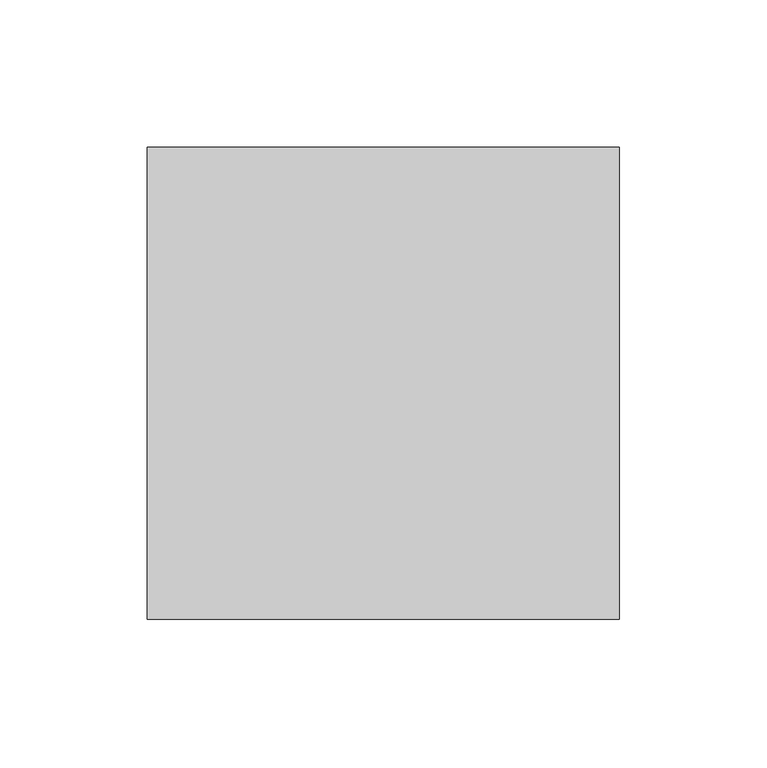
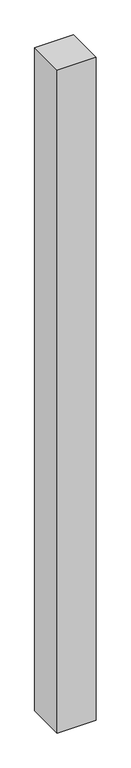
"""IFC4 building model written with IfcOpenShell, lengths in millimetres: proxy geometry, erzj."""

from ifc_helpers import new_model, si_unit, origin, origin_with_axes, place, context, project, spatial, polyline, outline, extrude, source, transform, mapped, element, save


def generic_models_d51feb7b(model_context):
    return source(origin(), model_context, "Body", "SweptSolid", [
        extrude(outline(polyline([(172678.7593015, 34594.7962965), (172678.7593015, 34434.7962965), (172518.7593015, 34434.7962965), (172518.7593015, 34594.7962965), (172678.7593015, 34594.7962965)])), origin_with_axes(), (0.0, 0.0, 1.0), 2880.0),
    ])


if __name__ == "__main__":
    model = new_model("IFC4")
    model_context = context("Model", 3, world=origin())
    ifc_project = project(units=[si_unit("LENGTHUNIT", "METRE", prefix="MILLI")], contexts=[model_context])
    site = spatial("IfcSite", under=ifc_project)
    building = spatial("IfcBuilding", under=site)
    placement = place(None, origin())
    generic_models_shape = generic_models_d51feb7b(model_context)
    element("IfcBuildingElementProxy", 1, Name="erzj", ObjectType="erzj", at=placement, inside=building, context=model_context, shape_type="MappedRepresentation", body=[
        mapped(generic_models_shape, transform((0.0, 0.0, 0.0), x_axis=(1.0, 0.0, 0.0), y_axis=(0.0, 1.0, 0.0), z_axis=(0.0, 0.0, 1.0))),
    ])
    save(model, "model.ifc")

# Revit data of these elements
# Element 1 (IfcBuildingElementProxy, "erzj")
#   Materials on its faces: "material wardrobe b 1"
# Materials
#   "material wardrobe b 1": class "Unassigned", colour RGB 128 128 128, transparency 0
